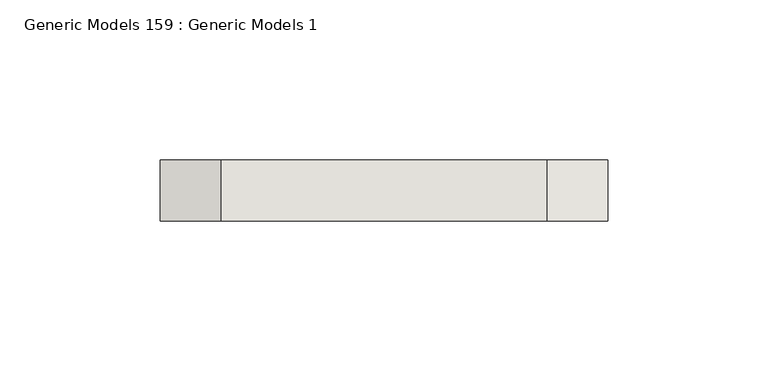
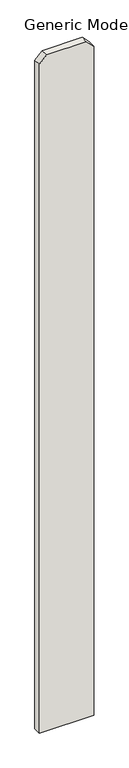
"""IFC4 building model written with IfcOpenShell, lengths in millimetres: wall geometry, Generic Models 159 : Generic Models 1."""

from ifc_helpers import new_model, si_unit, frame, origin, place, context, project, spatial, polyline, outline, extrude, source, transform, mapped, element, save


def generic_models_159_generic_models_1_ce90455c(model_context):
    return source(origin(), model_context, "Body", "SweptSolid", [
        extrude(outline(polyline([(76.2, 323213.4125), (1885.95, 323213.4125), (1905.0, 323194.3625), (1905.0, 323092.7625), (1885.95, 323073.7125), (76.2, 323073.7125), (76.2, 323213.4125)])), frame((0.0, 547.6875, 0.0), z_axis=(0.0, 1.0, 0.0), x_axis=(0.0, 0.0, 1.0)), (0.0, 0.0, 1.0), 19.05),
    ])


if __name__ == "__main__":
    model = new_model("IFC4")
    model_context = context("Model", 3, world=origin())
    ifc_project = project(units=[si_unit("LENGTHUNIT", "METRE", prefix="MILLI")], contexts=[model_context])
    site = spatial("IfcSite", under=ifc_project)
    building = spatial("IfcBuilding", under=site)
    placement = place(None, origin())
    generic_models_159_generic_models_1_shape = generic_models_159_generic_models_1_ce90455c(model_context)
    element("IfcWall", 1, ObjectType="Generic Models 159 : Generic Models 1", at=placement, inside=building, context=model_context, shape_type="MappedRepresentation", body=[
        mapped(generic_models_159_generic_models_1_shape, transform((0.0, 0.0, 0.0), x_axis=(1.0, 0.0, 0.0), y_axis=(0.0, 1.0, 0.0), z_axis=(0.0, 0.0, 1.0))),
    ])
    save(model, "model.ifc")

# Revit data of these elements
# Element 1 (IfcWall, "Generic Models 159 : Generic Models 1")
#   Materials on its faces: "VERTICAL 1X6 CEDAR PLANKS W/ CLEAR WOOD SEALER"
# Materials
#   "VERTICAL 1X6 CEDAR PLANKS W/ CLEAR WOOD SEALER": class "Wood", colour RGB 234 198 147, transparency 0, Description = "Pinus Echinata", Cost = 0
